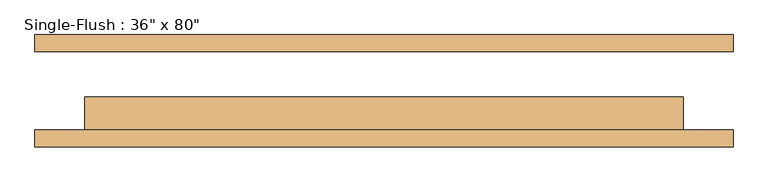
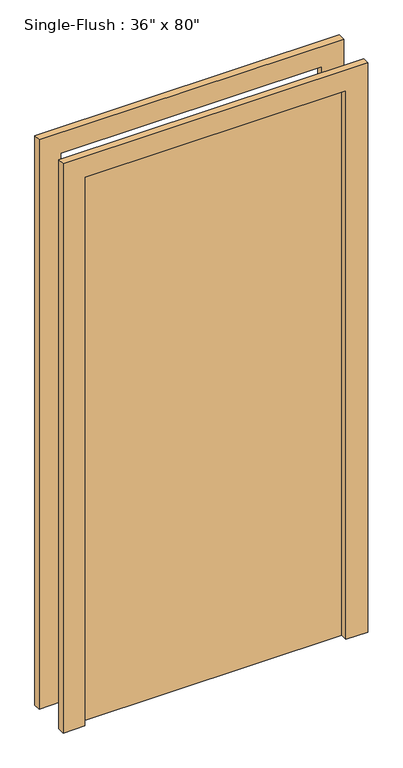
"""IFC4 building model written with IfcOpenShell, lengths in millimetres: door geometry."""

import ifcopenshell
import ifcopenshell.guid

model = None  # the IFC model being written
_history = None  # IfcOwnerHistory: only IFC2X3 demands one
_inside = {}  # id of a spatial element -> (the spatial element, [elements in it])
_under = {}  # id of a project, library or spatial element -> (it, [spatial elements below it])
_declared = {}  # id of a project -> (the project, [libraries it declares])
_typed = {}  # id of a type object -> (the type object, [elements of that type])
_made_of = {}  # id of a material, layer set ... -> (it, [elements and type objects made of it])


def new_model(schema):
    """Start an empty IFC model of exactly this schema.

    Asked for "IFC4X3", IfcOpenShell would pick the latest addendum, in which some entities
    have other attributes; the version numbers below select the first issue.
    IFC2X3 requires an IfcOwnerHistory on every rooted entity: one is made here for all.
    """
    global model, _history
    if schema == "IFC4X3":
        model = ifcopenshell.file(schema_version=(4, 3, 0, 0))
    else:
        model = ifcopenshell.file(schema=schema)
    _inside.clear()
    _under.clear()
    _declared.clear()
    _typed.clear()
    _made_of.clear()
    _history = None
    if model.schema == "IFC2X3":
        org = make("IfcOrganization", Name="unknown")
        user = make(
            "IfcPersonAndOrganization",
            ThePerson=make("IfcPerson", FamilyName="unknown"),
            TheOrganization=org,
        )
        app = make(
            "IfcApplication",
            ApplicationDeveloper=org,
            Version="unknown",
            ApplicationFullName="unknown",
            ApplicationIdentifier="unknown",
        )
        _history = make(
            "IfcOwnerHistory",
            OwningUser=user,
            OwningApplication=app,
            ChangeAction="ADDED",
            CreationDate=0,
        )
    return model


def make(cls, **values):
    """One entity of the class cls with the attributes given. An attribute that is None is left unset."""
    return model.create_entity(
        cls, **{name: value for name, value in values.items() if value is not None}
    )


def rooted(cls, **values):
    """An entity with a GlobalId (a new one), such as an element, a storey or a relation."""
    return make(cls, GlobalId=ifcopenshell.guid.new(), OwnerHistory=_history, **values)


def si_unit(unit_type, name, prefix=None):
    """IfcSIUnit, for example si_unit("LENGTHUNIT", "METRE", prefix="MILLI")."""
    return make("IfcSIUnit", UnitType=unit_type, Prefix=prefix, Name=name)


def assignment(units):
    """IfcUnitAssignment: the units of a project."""
    return None if units is None else make("IfcUnitAssignment", Units=units)


def point(xyz):
    """IfcCartesianPoint."""
    return None if xyz is None else make("IfcCartesianPoint", Coordinates=xyz)


def direction(xyz):
    """IfcDirection."""
    return None if xyz is None else make("IfcDirection", DirectionRatios=xyz)


def frame(location, z_axis=None, x_axis=None):
    """IfcAxis2Placement3D, a coordinate frame: its origin and axes. An axis left out is left unset."""
    return make(
        "IfcAxis2Placement3D",
        Location=point(location),
        Axis=direction(z_axis),
        RefDirection=direction(x_axis),
    )


def origin():
    """The frame at (0, 0, 0) with its axes left unset."""
    return frame((0.0, 0.0, 0.0))


def origin_with_axes():
    """The frame at (0, 0, 0) with the z axis (0, 0, 1) and the x axis (1, 0, 0) written out."""
    return frame((0.0, 0.0, 0.0), z_axis=(0.0, 0.0, 1.0), x_axis=(1.0, 0.0, 0.0))


def place(relative_to, where):
    """IfcLocalPlacement: puts the frame where relative to a parent placement (None: the world)."""
    return make(
        "IfcLocalPlacement", PlacementRelTo=relative_to, RelativePlacement=where
    )


def context(
    kind, dimensions, precision=None, world=None, true_north=None, identifier=None
):
    """IfcGeometricRepresentationContext, for example the 3D "Model" context."""
    return make(
        "IfcGeometricRepresentationContext",
        ContextIdentifier=identifier,
        ContextType=kind,
        CoordinateSpaceDimension=dimensions,
        Precision=precision,
        WorldCoordinateSystem=world,
        TrueNorth=true_north,
    )


def project(units=None, contexts=None):
    """IfcProject with its units and contexts."""
    return rooted(
        "IfcProject",
        Name="project",
        RepresentationContexts=contexts,
        UnitsInContext=assignment(units),
    )


def spatial(cls, under=None, at=None, **own):
    """A site, building, storey or space (cls), placed at a placement, below another one or the project."""
    s = rooted(cls, ObjectPlacement=at, **own)
    if under is not None:
        _under.setdefault(under.id(), (under, []))[1].append(s)
    return s


def polyline(points):
    """IfcPolyline through the points."""
    return make("IfcPolyline", Points=[point(p) for p in points])


def outline(outer, holes=None, kind="AREA"):
    """IfcArbitraryClosedProfileDef: a profile drawn as a closed curve; with holes, ...WithVoids."""
    if holes is None:
        return make("IfcArbitraryClosedProfileDef", ProfileType=kind, OuterCurve=outer)
    return make(
        "IfcArbitraryProfileDefWithVoids",
        ProfileType=kind,
        OuterCurve=outer,
        InnerCurves=holes,
    )


def extrude(swept, where, along, depth):
    """IfcExtrudedAreaSolid: the profile swept, set in the frame where, extruded along a direction by depth."""
    return make(
        "IfcExtrudedAreaSolid",
        SweptArea=swept,
        Position=where,
        ExtrudedDirection=direction(along),
        Depth=depth,
    )


def shape(context_of_items, identifier, shape_type, items):
    """IfcShapeRepresentation: the items that make up one representation, for example the "Body"."""
    return make(
        "IfcShapeRepresentation",
        ContextOfItems=context_of_items,
        RepresentationIdentifier=identifier,
        RepresentationType=shape_type,
        Items=items,
    )


def source(mapping_origin, context_of_items, identifier, shape_type, items):
    """IfcRepresentationMap: a shape defined once, which mapped items show again and again."""
    return make(
        "IfcRepresentationMap",
        MappingOrigin=mapping_origin,
        MappedRepresentation=shape(context_of_items, identifier, shape_type, items),
    )


def transform(
    local_origin,
    x_axis=None,
    y_axis=None,
    z_axis=None,
    scale=None,
    scale2=None,
    scale3=None,
    uniform=True,
):
    """IfcCartesianTransformationOperator3D, or its non-uniform kind. x_axis, y_axis, z_axis: its Axis1, 2, 3."""
    if uniform:
        return make(
            "IfcCartesianTransformationOperator3D",
            Axis1=direction(x_axis),
            Axis2=direction(y_axis),
            LocalOrigin=point(local_origin),
            Scale=scale,
            Axis3=direction(z_axis),
        )
    return make(
        "IfcCartesianTransformationOperator3DnonUniform",
        Axis1=direction(x_axis),
        Axis2=direction(y_axis),
        LocalOrigin=point(local_origin),
        Scale=scale,
        Axis3=direction(z_axis),
        Scale2=scale2,
        Scale3=scale3,
    )


def mapped(mapping_source, mapping_target):
    """IfcMappedItem: shows the shape of a source again, moved by a transform."""
    return make(
        "IfcMappedItem", MappingSource=mapping_source, MappingTarget=mapping_target
    )


def made_of(thing, what):
    """Note that an element or type object is made of a material, layer set ...; save() writes the relation."""
    if what is not None:
        _made_of.setdefault(what.id(), (what, []))[1].append(thing)
    return thing


def element(
    cls,
    number,
    at=None,
    inside=None,
    cuts=None,
    type_object=None,
    material=None,
    context=None,
    identifier="Body",
    shape_type=None,
    held_by="IfcProductDefinitionShape",
    body=None,
    shapes=None,
    **own,
):
    """One element of the class cls, such as IfcWall. Its Tag is "e" and its number.

    at: its placement. inside: the storey or other place that contains it. cuts: it is an
    opening in that element (IfcRelVoidsElement). A single representation is given by context,
    identifier, shape_type and body (its items); several are given by shapes. held_by: the class
    of the entity that holds the representations. save() writes the other relations.
    """
    e = rooted(cls, Tag="e%d" % number, ObjectPlacement=at, **own)
    if body is not None:
        shapes = [shape(context, identifier, shape_type, body)]
    if shapes is not None:
        e.Representation = make(held_by, Representations=shapes)
    if inside is not None:
        _inside.setdefault(inside.id(), (inside, []))[1].append(e)
    if cuts is not None:
        rooted(
            "IfcRelVoidsElement", RelatingBuildingElement=cuts, RelatedOpeningElement=e
        )
    if type_object is not None:
        _typed.setdefault(type_object.id(), (type_object, []))[1].append(e)
    return made_of(e, material)


def aggregate(whole, parts):
    """IfcRelAggregates: a whole, such as a stair, and the parts it consists of."""
    return rooted("IfcRelAggregates", RelatingObject=whole, RelatedObjects=parts)


def save(model, path):
    """Write the relations noted so far, then the file.

    IfcRelAggregates (storeys below a building ...), IfcRelContainedInSpatialStructure (elements
    in a storey), IfcRelDefinesByType, IfcRelAssociatesMaterial and IfcRelDeclares: one each for
    every whole, place, type object, material and project.
    """
    for whole, parts in _under.values():
        aggregate(whole, parts)
    for where, things in _inside.values():
        rooted(
            "IfcRelContainedInSpatialStructure",
            RelatedElements=things,
            RelatingStructure=where,
        )
    for kind, things in _typed.values():
        rooted("IfcRelDefinesByType", RelatedObjects=things, RelatingType=kind)
    for what, things in _made_of.values():
        rooted("IfcRelAssociatesMaterial", RelatedObjects=things, RelatingMaterial=what)
    for by, libraries in _declared.values():
        rooted("IfcRelDeclares", RelatingContext=by, RelatedDefinitions=libraries)
    model.write(path)


def door_bbe2d7fb(model_context):
    return source(origin(), model_context, "Body", "SweptSolid", [
        extrude(outline(polyline([(2108.2, -533.4), (0.0, -533.4), (0.0, -457.2), (2032.0, -457.2), (2032.0, 457.2), (0.0, 457.2), (0.0, 533.4), (2108.2, 533.4), (2108.2, -533.4)])), frame((0.0, -85.725, 0.0), z_axis=(0.0, 1.0, 0.0), x_axis=(0.0, 0.0, 1.0)), (0.0, 0.0, 1.0), 25.4),
        extrude(outline(polyline([(2108.2, 533.4), (2108.2, -533.4), (0.0, -533.4), (0.0, -457.2), (2032.0, -457.2), (2032.0, 457.2), (0.0, 457.2), (0.0, 533.4), (2108.2, 533.4)])), frame((0.0, 60.325, 0.0), z_axis=(0.0, 1.0, 0.0), x_axis=(0.0, 0.0, 1.0)), (0.0, 0.0, 1.0), 25.4),
        extrude(outline(polyline([(457.2, -9.525), (457.2, -60.325), (-457.2, -60.325), (-457.2, -9.525), (457.2, -9.525)])), origin_with_axes(), (0.0, 0.0, 1.0), 2032.0),
    ])


if __name__ == "__main__":
    model = new_model("IFC4")
    model_context = context("Model", 3, world=origin())
    ifc_project = project(units=[si_unit("LENGTHUNIT", "METRE", prefix="MILLI")], contexts=[model_context])
    site = spatial("IfcSite", under=ifc_project)
    building = spatial("IfcBuilding", under=site)
    placement = place(None, origin())
    door_shape = door_bbe2d7fb(model_context)
    element("IfcDoor", 1, ObjectType="Single-Flush : 36\" x 80\"", at=placement, inside=building, context=model_context, shape_type="MappedRepresentation", body=[
        mapped(door_shape, transform((0.0, 0.0, 0.0), x_axis=(1.0, 0.0, 0.0), y_axis=(0.0, 1.0, 0.0), z_axis=(0.0, 0.0, 1.0))),
    ])
    save(model, "model.ifc")

# Revit data of these elements
# Type "Single-Flush : 36\" x 80\""
#   Type Mark = "04"
#   Assembly Code = "C1020"
#   Thickness = 0' - 2"
#   Height = 6' - 8"
#   Trim Projection Ext = 0' - 1"
#   Trim Projection Int = 0' - 1"
#   Trim Width = 0' - 3"
#   Width = 3' - 0"
#   Door Material = drywall
#   Frame Material = drywall
#   Function = (empty or 0)
#   Wall Closure = (empty or 0)
# Element 1 (IfcDoor, "Single-Flush : 36\" x 80\"")
#   Materials on its faces: "drywall"
# Materials
#   "drywall": class "Generic", colour RGB 255 255 255, transparency 0, Description = "Gypsum Wall Board", Cost = 0
